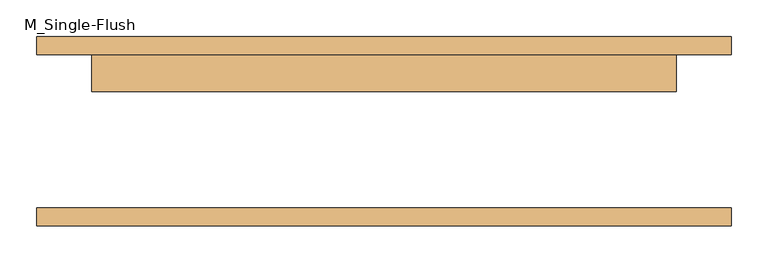
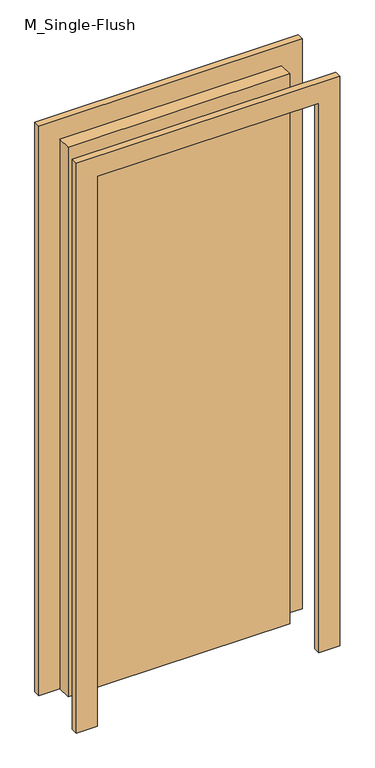
"""IFC4 building model written with IfcOpenShell, lengths in millimetres: door geometry, M_Single-Flush : 90x210cm Kapı."""

from ifc_helpers import new_model, si_unit, frame, origin, origin_with_axes, place, context, project, spatial, polyline, outline, extrude, source, transform, mapped, element, save


def m_single_flush_43d1bd44(model_context):
    return source(origin(), model_context, "Body", "SweptSolid", [
        extrude(outline(polyline([(2176.0, -476.0), (0.0, -476.0), (0.0, -400.0), (2100.0, -400.0), (2100.0, 400.0), (0.0, 400.0), (0.0, 476.0), (2176.0, 476.0), (2176.0, -476.0)])), frame((0.0, 105.0, 0.0), z_axis=(0.0, 1.0, 0.0), x_axis=(0.0, 0.0, 1.0)), (0.0, 0.0, 1.0), 25.0),
        extrude(outline(polyline([(2176.0, 476.0), (2176.0, -476.0), (0.0, -476.0), (0.0, -400.0), (2100.0, -400.0), (2100.0, 400.0), (0.0, 400.0), (0.0, 476.0), (2176.0, 476.0)])), frame((0.0, -130.0, 0.0), z_axis=(0.0, 1.0, 0.0), x_axis=(0.0, 0.0, 1.0)), (0.0, 0.0, 1.0), 25.0),
        extrude(outline(polyline([(400.0, 54.0), (-400.0, 54.0), (-400.0, 105.0), (400.0, 105.0), (400.0, 54.0)])), origin_with_axes(), (0.0, 0.0, 1.0), 2100.0),
    ])


if __name__ == "__main__":
    model = new_model("IFC4")
    model_context = context("Model", 3, world=origin())
    ifc_project = project(units=[si_unit("LENGTHUNIT", "METRE", prefix="MILLI")], contexts=[model_context])
    site = spatial("IfcSite", under=ifc_project)
    building = spatial("IfcBuilding", under=site)
    placement = place(None, origin())
    m_single_flush_shape = m_single_flush_43d1bd44(model_context)
    element("IfcDoor", 1, ObjectType="M_Single-Flush : 90x210cm Kapı", at=placement, inside=building, context=model_context, shape_type="MappedRepresentation", body=[
        mapped(m_single_flush_shape, transform((0.0, 0.0, 0.0), x_axis=(1.0, 0.0, 0.0), y_axis=(0.0, 1.0, 0.0), z_axis=(0.0, 0.0, 1.0))),
    ])
    save(model, "model.ifc")

# Revit data of these elements
# Type "M_Single-Flush : 90x210cm Kapı"
#   Type Mark = "40"
#   Construction Type Id = "MDOOR"
#   Analytic Construction = "Metal"
#   Thickness = 5.10 cm
#   Heat Transfer Coefficient (U) = 3.7021 W/(m²·K)
#   Height = 210.00 cm
#   Trim Projection Ext = 2.50 cm
#   Trim Projection Int = 2.50 cm
#   Trim Width = 7.60 cm
#   Width = 80.00 cm
#   Define Thermal Properties by = 1
#   Door Material = Door - Panel
#   Frame Material = Door - Frame
#   Visual Light Transmittance = 0
#   Solar Heat Gain Coefficient = 0
#   Function = (empty or 0)
#   Wall Closure = (empty or 0)
# Element 1 (IfcDoor, "M_Single-Flush : 90x210cm Kapı")
#   Materials on its faces: "Door - Frame", "Door - Panel"
# Materials
#   "Door - Panel": class "Wood", colour RGB 210 159 95, transparency 0
#   "Door - Frame": class "Miscellaneous", colour RGB 118 70 51, transparency 0
